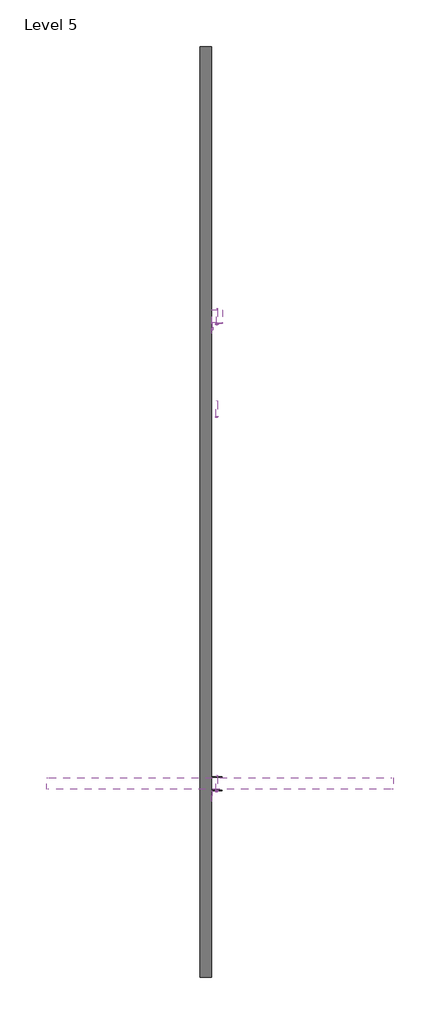
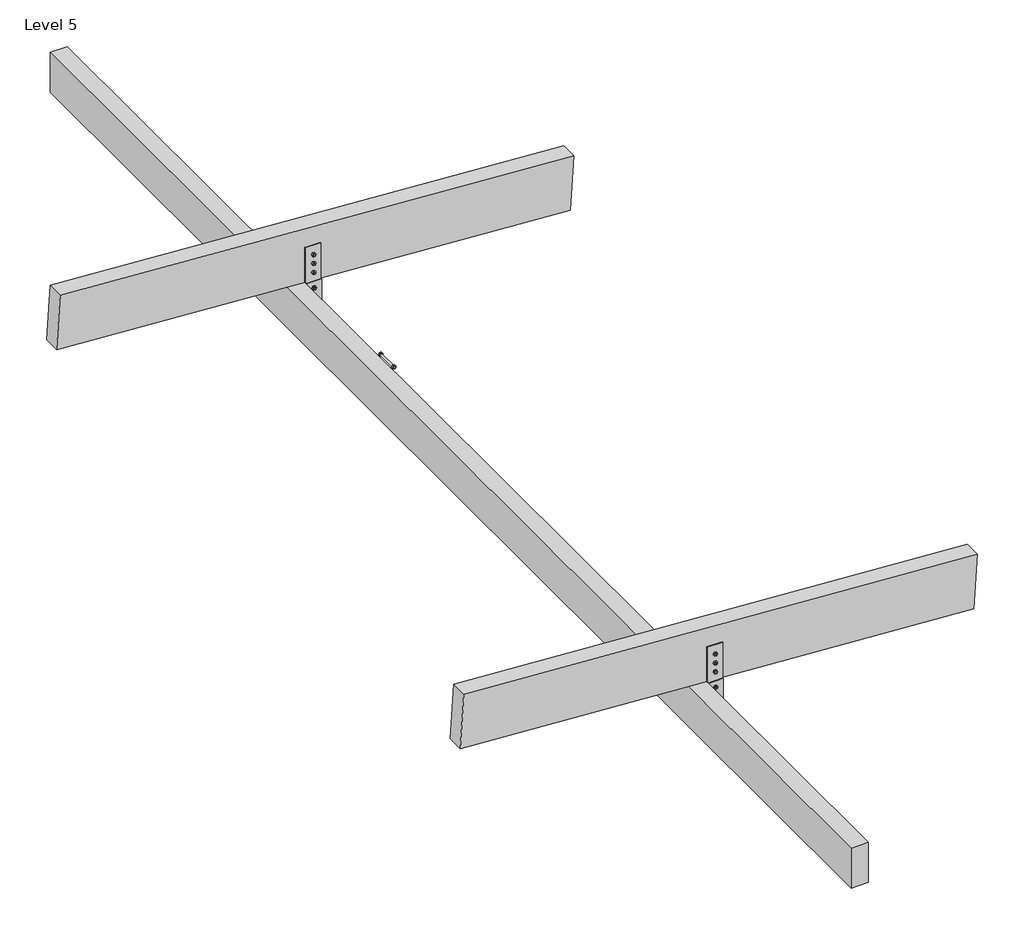
# One storey: 43 proxies.
# Revit data of these elements (continued)
# Project information
#   Project Issue Date = "Issue Date"
#   Project Status = "Project Status"
#   Client Name = "Owner"
#   Project Address = "640 West Main Street, Lake Geneva, WI 53147"
#   Project Name = "The Downtowner"
#   Project Number = "Project Number"
# Type "ROD : ROD"
#   lenght = 0' - 7 1/4"
#   Radius = 0' - 0 41/128"
#   material [instance default] = 3/4" GALV. THRU BOLTS
# Type "ROD : ROD 8"
#   lenght = 0' - 8"
#   Radius = 0' - 0 41/128"
#   material [instance default] = 3/4" GALV. THRU BOLTS
# Element 1 (IfcBuildingElementProxy, "Generic Models 108 : Generic Models 73")
#   Phase Created = New Construction
#   Materials on its faces: "5/16 GALV. PLATE"
# Element 2 (IfcBuildingElementProxy, "Generic Models 142 : Generic Models 75")
#   Phase Created = New Construction
#   Materials on its faces: "3/4\" GALV. THRU BOLTS"
# Element 3 (IfcBuildingElementProxy, "Generic Models 155 : Generic Models 75")
#   Phase Created = New Construction
#   Materials on its faces: "3/4\" GALV. THRU BOLTS"
# Element 4 (IfcBuildingElementProxy, "Generic Models 166 : Generic Models 73")
#   Phase Created = New Construction
#   Materials on its faces: "5/16\" THICK GALV. STEEL PLATE", "5/16 THICK GALV. SADDLE"
# Element 5 (IfcBuildingElementProxy, "Generic Models 168 : Generic Models 75")
#   Phase Created = New Construction
#   Materials on its faces: "3/4\" GALV. THRU BOLTS"
# Element 6 (IfcBuildingElementProxy, "Generic Models 172 : Generic Models 70")
#   Transparency Hack = "Yes"
#   Phase Created = New Construction
#   Materials on its faces: "5 1/2\" x 18\" GLULAM BEAM"
# Element 7 (IfcBuildingElementProxy, "Generic Models 173 : Generic Models 75")
#   Phase Created = New Construction
#   Materials on its faces: "3/4\" GALV. THRU BOLTS"
# Element 8 (IfcBuildingElementProxy, "Generic Models 174 : Generic Models 75")
#   Phase Created = New Construction
#   Materials on its faces: "3/4\" GALV. THRU BOLTS"
# Element 9 (IfcBuildingElementProxy, "Generic Models 175 : Generic Models 75")
#   Phase Created = New Construction
#   Materials on its faces: "3/4\" GALV. THRU BOLTS"
# Element 10 (IfcBuildingElementProxy, "Generic Models 176 : Generic Models 75")
#   Phase Created = New Construction
#   Materials on its faces: "3/4\" GALV. THRU BOLTS"
# Element 11 (IfcBuildingElementProxy, "Generic Models 179 : Generic Models 75")
#   Phase Created = New Construction
#   Materials on its faces: "3/4\" GALV. THRU BOLTS"
# Element 12 (IfcBuildingElementProxy, "Generic Models 197 : Generic Models 75")
#   Phase Created = New Construction
#   Materials on its faces: "3/4\" GALV. THRU BOLTS"
# Element 13 (IfcBuildingElementProxy, "Generic Models 199 : Generic Models 75")
#   Phase Created = New Construction
#   Materials on its faces: "3/4\" GALV. THRU BOLTS"
# Element 14 (IfcBuildingElementProxy, "Generic Models 203 : Generic Models 75")
#   Phase Created = New Construction
#   Materials on its faces: "3/4\" DIA LAG BOLTS"
# Element 15 (IfcBuildingElementProxy, "Generic Models 207 : Generic Models 75")
#   Phase Created = New Construction
#   Materials on its faces: "3/4\" GALV. THRU BOLTS"
# Element 16 (IfcBuildingElementProxy, "Generic Models 211 : Generic Models 75")
#   Phase Created = New Construction
#   Materials on its faces: "3/4\" GALV. THRU BOLTS"
# Element 17 (IfcBuildingElementProxy, "Generic Models 239 : Generic Models 75")
#   Phase Created = New Construction
#   Materials on its faces: "3/4\" GALV. THRU BOLTS"
# Element 18 (IfcBuildingElementProxy, "Generic Models 272 : Generic Models 73")
#   Phase Created = New Construction
#   Materials on its faces: "5/16 GALV. PLATE"
# Element 19 (IfcBuildingElementProxy, "Generic Models 70 : Generic Models 70")
#   Phase Created = New Construction
#   Materials on its faces: "5 1/2\" x 13 1/2\" GLUELAM BEAM"
# Element 20 (IfcBuildingElementProxy, "Generic Models 73 : Generic Models 73")
#   Phase Created = New Construction
#   Materials on its faces: "5/16\" THICK GALV. STEEL PLATE", "5/16 THICK GALV. SADDLE"
# Element 21 (IfcBuildingElementProxy, "Generic Models 78 : Generic Models 75")
#   Phase Created = New Construction
#   Materials on its faces: "3/4\" GALV. THRU BOLTS"
# Element 22 (IfcBuildingElementProxy, "Generic Models 79 : Generic Models 75")
#   Phase Created = New Construction
#   Materials on its faces: "3/4\" GALV. THRU BOLTS"
# Elements 23, 24, 25, 26, 27, 28, 29, 30, 31 (IfcBuildingElementProxy, "ROD : ROD")
#   material = 3/4" GALV. THRU BOLTS
#   Phase Created = New Construction
# Elements 32, 33, 34, 35, 36, 37, 38, 39, 40, 41, 42 (IfcBuildingElementProxy, "ROD : ROD 8")
#   material = 3/4" GALV. THRU BOLTS
#   Phase Created = New Construction
# Element 43 (IfcBuildingElementProxy, "ROD : ROD 8")
#   Phase Created = New Construction
# Materials
#   "3/4\" GALV. THRU BOLTS": class "Generic", colour RGB 105 69 171, transparency 0, Cost = 0
#   "5/16 GALV. PLATE": class "Metal", colour RGB 199 199 199, transparency 0, Description = "Carbon steel", Cost = 0
#   "5/16\" THICK GALV. STEEL PLATE": class "Metal", colour RGB 199 199 199, transparency 0, Description = "Carbon steel", Cost = 0
#   "5/16 THICK GALV. SADDLE": class "Metal", colour RGB 199 199 199, transparency 0, Description = "Carbon steel", Cost = 0
#   "5 1/2\" x 18\" GLULAM BEAM": class "Wood", colour RGB 112 64 44, transparency 0, Description = "Pinus Echinata", Cost = 0
#   "3/4\" DIA LAG BOLTS": class "Generic", colour RGB 255 255 0, transparency 0, Cost = 0
#   "5 1/2\" x 13 1/2\" GLUELAM BEAM": class "Wood", colour RGB 211 164 143, transparency 0, Description = "Pinus Echinata", Cost = 0
